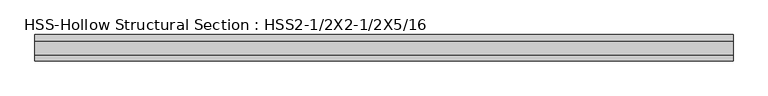
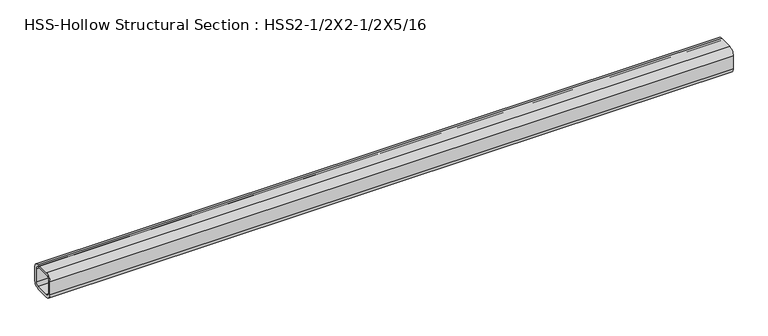
"""IFC4 building model written with IfcOpenShell, lengths in millimetres: beam geometry, HSS-Hollow Structural Section : HSS2-1/2X2-1/2X5/16."""

import ifcopenshell
import ifcopenshell.guid

model = None  # the IFC model being written
_history = None  # IfcOwnerHistory: only IFC2X3 demands one
_inside = {}  # id of a spatial element -> (the spatial element, [elements in it])
_under = {}  # id of a project, library or spatial element -> (it, [spatial elements below it])
_declared = {}  # id of a project -> (the project, [libraries it declares])
_typed = {}  # id of a type object -> (the type object, [elements of that type])
_made_of = {}  # id of a material, layer set ... -> (it, [elements and type objects made of it])


def new_model(schema):
    """Start an empty IFC model of exactly this schema.

    Asked for "IFC4X3", IfcOpenShell would pick the latest addendum, in which some entities
    have other attributes; the version numbers below select the first issue.
    IFC2X3 requires an IfcOwnerHistory on every rooted entity: one is made here for all.
    """
    global model, _history
    if schema == "IFC4X3":
        model = ifcopenshell.file(schema_version=(4, 3, 0, 0))
    else:
        model = ifcopenshell.file(schema=schema)
    _inside.clear()
    _under.clear()
    _declared.clear()
    _typed.clear()
    _made_of.clear()
    _history = None
    if model.schema == "IFC2X3":
        org = make("IfcOrganization", Name="unknown")
        user = make(
            "IfcPersonAndOrganization",
            ThePerson=make("IfcPerson", FamilyName="unknown"),
            TheOrganization=org,
        )
        app = make(
            "IfcApplication",
            ApplicationDeveloper=org,
            Version="unknown",
            ApplicationFullName="unknown",
            ApplicationIdentifier="unknown",
        )
        _history = make(
            "IfcOwnerHistory",
            OwningUser=user,
            OwningApplication=app,
            ChangeAction="ADDED",
            CreationDate=0,
        )
    return model


def make(cls, **values):
    """One entity of the class cls with the attributes given. An attribute that is None is left unset."""
    return model.create_entity(
        cls, **{name: value for name, value in values.items() if value is not None}
    )


def rooted(cls, **values):
    """An entity with a GlobalId (a new one), such as an element, a storey or a relation."""
    return make(cls, GlobalId=ifcopenshell.guid.new(), OwnerHistory=_history, **values)


def si_unit(unit_type, name, prefix=None):
    """IfcSIUnit, for example si_unit("LENGTHUNIT", "METRE", prefix="MILLI")."""
    return make("IfcSIUnit", UnitType=unit_type, Prefix=prefix, Name=name)


def assignment(units):
    """IfcUnitAssignment: the units of a project."""
    return None if units is None else make("IfcUnitAssignment", Units=units)


def point(xyz):
    """IfcCartesianPoint."""
    return None if xyz is None else make("IfcCartesianPoint", Coordinates=xyz)


def direction(xyz):
    """IfcDirection."""
    return None if xyz is None else make("IfcDirection", DirectionRatios=xyz)


def frame(location, z_axis=None, x_axis=None):
    """IfcAxis2Placement3D, a coordinate frame: its origin and axes. An axis left out is left unset."""
    return make(
        "IfcAxis2Placement3D",
        Location=point(location),
        Axis=direction(z_axis),
        RefDirection=direction(x_axis),
    )


def frame_2d(location, x_axis=None):
    """IfcAxis2Placement2D, a coordinate frame in the plane: its origin and x axis."""
    return make(
        "IfcAxis2Placement2D", Location=point(location), RefDirection=direction(x_axis)
    )


def origin():
    """The frame at (0, 0, 0) with its axes left unset."""
    return frame((0.0, 0.0, 0.0))


def place(relative_to, where):
    """IfcLocalPlacement: puts the frame where relative to a parent placement (None: the world)."""
    return make(
        "IfcLocalPlacement", PlacementRelTo=relative_to, RelativePlacement=where
    )


def context(
    kind, dimensions, precision=None, world=None, true_north=None, identifier=None
):
    """IfcGeometricRepresentationContext, for example the 3D "Model" context."""
    return make(
        "IfcGeometricRepresentationContext",
        ContextIdentifier=identifier,
        ContextType=kind,
        CoordinateSpaceDimension=dimensions,
        Precision=precision,
        WorldCoordinateSystem=world,
        TrueNorth=true_north,
    )


def project(units=None, contexts=None):
    """IfcProject with its units and contexts."""
    return rooted(
        "IfcProject",
        Name="project",
        RepresentationContexts=contexts,
        UnitsInContext=assignment(units),
    )


def spatial(cls, under=None, at=None, **own):
    """A site, building, storey or space (cls), placed at a placement, below another one or the project."""
    s = rooted(cls, ObjectPlacement=at, **own)
    if under is not None:
        _under.setdefault(under.id(), (under, []))[1].append(s)
    return s


def polyline(points):
    """IfcPolyline through the points."""
    return make("IfcPolyline", Points=[point(p) for p in points])


def circle_curve(where, radius):
    """IfcCircle in the frame where."""
    return make("IfcCircle", Position=where, Radius=radius)


def trimmed(basis, trim1, trim2, sense, master):
    """IfcTrimmedCurve: the piece of a basis curve between two trims."""
    return make(
        "IfcTrimmedCurve",
        BasisCurve=basis,
        Trim1=trim1,
        Trim2=trim2,
        SenseAgreement=sense,
        MasterRepresentation=master,
    )


def segment(curve, same_sense, transition):
    """IfcCompositeCurveSegment."""
    return make(
        "IfcCompositeCurveSegment",
        Transition=transition,
        SameSense=same_sense,
        ParentCurve=curve,
    )


def composite_curve(segments, self_intersect=None):
    """IfcCompositeCurve: segments joined end to end."""
    return make("IfcCompositeCurve", Segments=segments, SelfIntersect=self_intersect)


def outline(outer, holes=None, kind="AREA"):
    """IfcArbitraryClosedProfileDef: a profile drawn as a closed curve; with holes, ...WithVoids."""
    if holes is None:
        return make("IfcArbitraryClosedProfileDef", ProfileType=kind, OuterCurve=outer)
    return make(
        "IfcArbitraryProfileDefWithVoids",
        ProfileType=kind,
        OuterCurve=outer,
        InnerCurves=holes,
    )


def extrude(swept, where, along, depth):
    """IfcExtrudedAreaSolid: the profile swept, set in the frame where, extruded along a direction by depth."""
    return make(
        "IfcExtrudedAreaSolid",
        SweptArea=swept,
        Position=where,
        ExtrudedDirection=direction(along),
        Depth=depth,
    )


def shape(context_of_items, identifier, shape_type, items):
    """IfcShapeRepresentation: the items that make up one representation, for example the "Body"."""
    return make(
        "IfcShapeRepresentation",
        ContextOfItems=context_of_items,
        RepresentationIdentifier=identifier,
        RepresentationType=shape_type,
        Items=items,
    )


def source(mapping_origin, context_of_items, identifier, shape_type, items):
    """IfcRepresentationMap: a shape defined once, which mapped items show again and again."""
    return make(
        "IfcRepresentationMap",
        MappingOrigin=mapping_origin,
        MappedRepresentation=shape(context_of_items, identifier, shape_type, items),
    )


def transform(
    local_origin,
    x_axis=None,
    y_axis=None,
    z_axis=None,
    scale=None,
    scale2=None,
    scale3=None,
    uniform=True,
):
    """IfcCartesianTransformationOperator3D, or its non-uniform kind. x_axis, y_axis, z_axis: its Axis1, 2, 3."""
    if uniform:
        return make(
            "IfcCartesianTransformationOperator3D",
            Axis1=direction(x_axis),
            Axis2=direction(y_axis),
            LocalOrigin=point(local_origin),
            Scale=scale,
            Axis3=direction(z_axis),
        )
    return make(
        "IfcCartesianTransformationOperator3DnonUniform",
        Axis1=direction(x_axis),
        Axis2=direction(y_axis),
        LocalOrigin=point(local_origin),
        Scale=scale,
        Axis3=direction(z_axis),
        Scale2=scale2,
        Scale3=scale3,
    )


def mapped(mapping_source, mapping_target):
    """IfcMappedItem: shows the shape of a source again, moved by a transform."""
    return make(
        "IfcMappedItem", MappingSource=mapping_source, MappingTarget=mapping_target
    )


def made_of(thing, what):
    """Note that an element or type object is made of a material, layer set ...; save() writes the relation."""
    if what is not None:
        _made_of.setdefault(what.id(), (what, []))[1].append(thing)
    return thing


def element(
    cls,
    number,
    at=None,
    inside=None,
    cuts=None,
    type_object=None,
    material=None,
    context=None,
    identifier="Body",
    shape_type=None,
    held_by="IfcProductDefinitionShape",
    body=None,
    shapes=None,
    **own,
):
    """One element of the class cls, such as IfcWall. Its Tag is "e" and its number.

    at: its placement. inside: the storey or other place that contains it. cuts: it is an
    opening in that element (IfcRelVoidsElement). A single representation is given by context,
    identifier, shape_type and body (its items); several are given by shapes. held_by: the class
    of the entity that holds the representations. save() writes the other relations.
    """
    e = rooted(cls, Tag="e%d" % number, ObjectPlacement=at, **own)
    if body is not None:
        shapes = [shape(context, identifier, shape_type, body)]
    if shapes is not None:
        e.Representation = make(held_by, Representations=shapes)
    if inside is not None:
        _inside.setdefault(inside.id(), (inside, []))[1].append(e)
    if cuts is not None:
        rooted(
            "IfcRelVoidsElement", RelatingBuildingElement=cuts, RelatedOpeningElement=e
        )
    if type_object is not None:
        _typed.setdefault(type_object.id(), (type_object, []))[1].append(e)
    return made_of(e, material)


def aggregate(whole, parts):
    """IfcRelAggregates: a whole, such as a stair, and the parts it consists of."""
    return rooted("IfcRelAggregates", RelatingObject=whole, RelatedObjects=parts)


def save(model, path):
    """Write the relations noted so far, then the file.

    IfcRelAggregates (storeys below a building ...), IfcRelContainedInSpatialStructure (elements
    in a storey), IfcRelDefinesByType, IfcRelAssociatesMaterial and IfcRelDeclares: one each for
    every whole, place, type object, material and project.
    """
    for whole, parts in _under.values():
        aggregate(whole, parts)
    for where, things in _inside.values():
        rooted(
            "IfcRelContainedInSpatialStructure",
            RelatedElements=things,
            RelatingStructure=where,
        )
    for kind, things in _typed.values():
        rooted("IfcRelDefinesByType", RelatedObjects=things, RelatingType=kind)
    for what, things in _made_of.values():
        rooted("IfcRelAssociatesMaterial", RelatedObjects=things, RelatingMaterial=what)
    for by, libraries in _declared.values():
        rooted("IfcRelDeclares", RelatingContext=by, RelatedDefinitions=libraries)
    model.write(path)


def hss_hollow_structural_section_hss2_1_2x2_1_2x5_16_8c771364(model_context):
    return source(origin(), model_context, "Body", "SweptSolid", [
        extrude(outline(composite_curve([segment(polyline([(31.75, 16.9672), (31.75, -16.9672)]), True, "CONTINUOUS"), segment(trimmed(circle_curve(frame_2d((16.9672, -16.9672)), 14.7828), [point((31.75, -16.9672))], [point((16.9672, -31.75))], False, "CARTESIAN"), True, "CONTINUOUS"), segment(polyline([(16.9672, -31.75), (-16.9672, -31.75)]), True, "CONTINUOUS"), segment(trimmed(circle_curve(frame_2d((-16.9672, -16.9672)), 14.7828), [point((-16.9672, -31.75))], [point((-31.75, -16.9672))], False, "CARTESIAN"), True, "CONTINUOUS"), segment(polyline([(-31.75, -16.9672), (-31.75, 16.9672)]), True, "CONTINUOUS"), segment(trimmed(circle_curve(frame_2d((-16.9672, 16.9672)), 14.7828), [point((-31.75, 16.9672))], [point((-16.9672, 31.75))], False, "CARTESIAN"), True, "CONTINUOUS"), segment(polyline([(-16.9672, 31.75), (16.9672, 31.75)]), True, "CONTINUOUS"), segment(trimmed(circle_curve(frame_2d((16.9672, 16.9672)), 14.7828), [point((16.9672, 31.75))], [point((31.75, 16.9672))], False, "CARTESIAN"), True, "CONTINUOUS")], self_intersect=False), holes=[composite_curve([segment(trimmed(circle_curve(frame_2d((-16.9672, 16.9672)), 7.3914), [point((-16.9672, 24.3586))], [point((-24.3586, 16.9672))], True, "CARTESIAN"), True, "CONTINUOUS"), segment(polyline([(-24.3586, 16.9672), (-24.3586, -16.9672)]), True, "CONTINUOUS"), segment(trimmed(circle_curve(frame_2d((-16.9672, -16.9672)), 7.3914), [point((-24.3586, -16.9672))], [point((-16.9672, -24.3586))], True, "CARTESIAN"), True, "CONTINUOUS"), segment(polyline([(-16.9672, -24.3586), (16.9672, -24.3586)]), True, "CONTINUOUS"), segment(trimmed(circle_curve(frame_2d((16.9672, -16.9672)), 7.3914), [point((16.9672, -24.3586))], [point((24.3586, -16.9672))], True, "CARTESIAN"), True, "CONTINUOUS"), segment(polyline([(24.3586, -16.9672), (24.3586, 16.9672)]), True, "CONTINUOUS"), segment(trimmed(circle_curve(frame_2d((16.9672, 16.9672)), 7.3914), [point((24.3586, 16.9672))], [point((16.9672, 24.3586))], True, "CARTESIAN"), True, "CONTINUOUS"), segment(polyline([(16.9672, 24.3586), (-16.9672, 24.3586)]), True, "CONTINUOUS")], self_intersect=False)]), frame((-835.5027583, 0.0, 0.0), z_axis=(1.0, 0.0, 0.0), x_axis=(0.0, 1.0, 0.0)), (0.0, 0.0, 1.0), 1671.0055167),
    ])


if __name__ == "__main__":
    model = new_model("IFC4")
    model_context = context("Model", 3, world=origin())
    ifc_project = project(units=[si_unit("LENGTHUNIT", "METRE", prefix="MILLI")], contexts=[model_context])
    site = spatial("IfcSite", under=ifc_project)
    building = spatial("IfcBuilding", under=site)
    placement = place(None, origin())
    hss_hollow_structural_section_hss2_1_2x2_1_2x5_16_shape = hss_hollow_structural_section_hss2_1_2x2_1_2x5_16_8c771364(model_context)
    element("IfcBeam", 1, ObjectType="HSS-Hollow Structural Section : HSS2-1/2X2-1/2X5/16", at=placement, inside=building, context=model_context, shape_type="MappedRepresentation", body=[
        mapped(hss_hollow_structural_section_hss2_1_2x2_1_2x5_16_shape, transform((0.0, 0.0, 0.0), x_axis=(1.0, 0.0, 0.0), y_axis=(0.0, 1.0, 0.0), z_axis=(0.0, 0.0, 1.0))),
    ])
    save(model, "model.ifc")

# Revit data of these elements
# Type "HSS-Hollow Structural Section : HSS2-1/2X2-1/2X5/16"
#   Assembly Code = "B10"
#   Shape = "Square"
#   W = 8.4
#   Ht = 0' - 2 1/2"
#   Length [instance default] = 5' - 0"
#   b = 0' - 2 1/2"
#   kr = 0' - 0.582"
#   t = 0' - 0.291"
#   A = 0.0163194 SF
#   Structural Material [instance default] = Steel ASTM A500, Grade B, Rectangular and Square
# Element 1 (IfcBeam, "HSS-Hollow Structural Section : HSS2-1/2X2-1/2X5/16")
#   Materials on its faces: "Steel ASTM A500, Grade B, Rectangular and Square"
# Materials
#   "Steel ASTM A500, Grade B, Rectangular and Square": class "Metal", colour RGB 199 199 199, transparency 0, Description = "Carbon steel", Cost = 0
